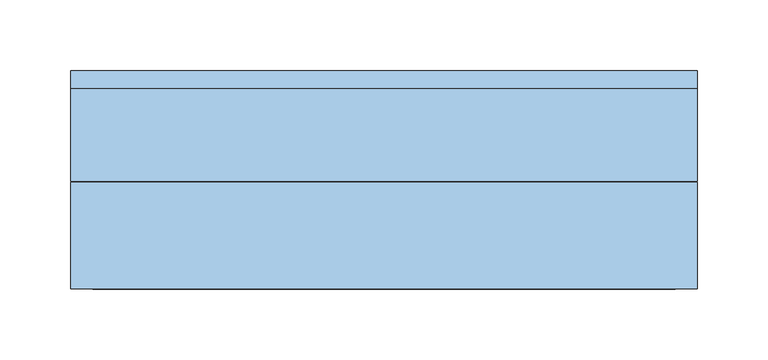
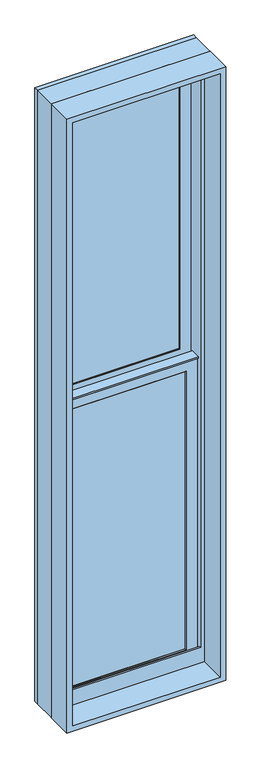
"""IFC4 building model written with IfcOpenShell, lengths in millimetres: window geometry, Window-Double_Hung-Marvin-Essential : ESDH1660."""

from ifc_helpers import new_model, si_unit, frame, origin, place, context, project, spatial, polyline, outline, extrude, faceted_brep, source, transform, mapped, element, save


def window_828d42fd(model_context):
    return source(origin(), model_context, "Body", "SolidModel", [
        extrude(outline(polyline([(64.5583333, 20.6375), (64.5583333, 15.875), (45.5083333, 15.875), (45.5083333, 20.6375), (64.5583333, 20.6375)])), frame((0.0, 0.0, 679.45), z_axis=(0.0, 0.0, 1.0), x_axis=(1.0, 0.0, 0.0)), (0.0, 0.0, 1.0), 831.85),
        extrude(outline(polyline([(-45.5083333, 20.6375), (-45.5083333, 15.875), (-64.5583333, 15.875), (-64.5583333, 20.6375), (-45.5083333, 20.6375)])), frame((0.0, 0.0, 679.45), z_axis=(0.0, 0.0, 1.0), x_axis=(1.0, 0.0, 0.0)), (0.0, 0.0, 1.0), 831.85),
        extrude(outline(polyline([(165.1, 20.6375), (165.1, 15.875), (-165.1, 15.875), (-165.1, 20.6375), (165.1, 20.6375)])), frame((0.0, 0.0, 1085.85), z_axis=(0.0, 0.0, 1.0), x_axis=(1.0, 0.0, 0.0)), (0.0, 0.0, 1.0), 19.05),
        extrude(outline(polyline([(-64.5583333, 46.83125), (-64.5583333, 51.59375), (-45.5083333, 51.59375), (-45.5083333, 46.83125), (-64.5583333, 46.83125)])), frame((0.0, 0.0, 1549.4), z_axis=(0.0, 0.0, 1.0), x_axis=(1.0, 0.0, 0.0)), (0.0, 0.0, 1.0), 831.85),
        extrude(outline(polyline([(45.5083333, 46.83125), (45.5083333, 51.59375), (64.5583333, 51.59375), (64.5583333, 46.83125), (45.5083333, 46.83125)])), frame((0.0, 0.0, 1549.4), z_axis=(0.0, 0.0, 1.0), x_axis=(1.0, 0.0, 0.0)), (0.0, 0.0, 1.0), 831.85),
        extrude(outline(polyline([(-165.1, 46.83125), (-165.1, 51.59375), (165.1, 51.59375), (165.1, 46.83125), (-165.1, 46.83125)])), frame((0.0, 0.0, 1955.8), z_axis=(0.0, 0.0, 1.0), x_axis=(1.0, 0.0, 0.0)), (0.0, 0.0, 1.0), 19.05),
        extrude(outline(polyline([(64.5583333, 20.6375), (45.5083333, 20.6375), (45.5083333, 25.4), (64.5583333, 25.4), (64.5583333, 20.6375)])), frame((0.0, 0.0, 679.45), z_axis=(0.0, 0.0, 1.0), x_axis=(1.0, 0.0, 0.0)), (0.0, 0.0, 1.0), 831.85),
        extrude(outline(polyline([(-45.5083333, 20.6375), (-64.5583333, 20.6375), (-64.5583333, 25.4), (-45.5083333, 25.4), (-45.5083333, 20.6375)])), frame((0.0, 0.0, 679.45), z_axis=(0.0, 0.0, 1.0), x_axis=(1.0, 0.0, 0.0)), (0.0, 0.0, 1.0), 831.85),
        extrude(outline(polyline([(165.1, 20.6375), (-165.1, 20.6375), (-165.1, 25.4), (165.1, 25.4), (165.1, 20.6375)])), frame((0.0, 0.0, 1085.85), z_axis=(0.0, 0.0, 1.0), x_axis=(1.0, 0.0, 0.0)), (0.0, 0.0, 1.0), 19.05),
        extrude(outline(polyline([(-64.5583333, 56.35625), (-45.5083333, 56.35625), (-45.5083333, 51.59375), (-64.5583333, 51.59375), (-64.5583333, 56.35625)])), frame((0.0, 0.0, 1549.4), z_axis=(0.0, 0.0, 1.0), x_axis=(1.0, 0.0, 0.0)), (0.0, 0.0, 1.0), 831.85),
        extrude(outline(polyline([(45.5083333, 56.35625), (64.5583333, 56.35625), (64.5583333, 51.59375), (45.5083333, 51.59375), (45.5083333, 56.35625)])), frame((0.0, 0.0, 1549.4), z_axis=(0.0, 0.0, 1.0), x_axis=(1.0, 0.0, 0.0)), (0.0, 0.0, 1.0), 831.85),
        extrude(outline(polyline([(-165.1, 56.35625), (165.1, 56.35625), (165.1, 51.59375), (-165.1, 51.59375), (-165.1, 56.35625)])), frame((0.0, 0.0, 1955.8), z_axis=(0.0, 0.0, 1.0), x_axis=(1.0, 0.0, 0.0)), (0.0, 0.0, 1.0), 19.05),
        faceted_brep([(-192.0875, 5.6780605, 1541.3351748), (-192.0875, 5.6780605, 1536.7), (192.0875, 5.6780605, 1536.7), (192.0875, 5.6780605, 1541.3351748), (-192.0875, 34.8118605, 1541.3351748), (192.0875, 34.8118605, 1541.3351748), (192.0875, 34.8118605, 1536.7), (-192.0875, 34.8118605, 1536.7), (-192.0875, 30.1625, 1536.7), (-192.0875, 30.1625, 652.4625), (-192.0875, 8.9241104, 652.4625), (-192.0875, 8.9241104, 1536.7), (192.0875, 8.9241104, 1536.7), (192.0875, 30.1625, 1536.7), (192.0875, 8.9241104, 652.4625), (192.0875, 30.1625, 652.4625), (-176.2034752, 11.90625, 1522.4034752), (-176.2034752, 30.1625, 1522.4034752), (176.2034752, 30.1625, 1522.4034752), (176.2034752, 11.90625, 1522.4034752), (-159.54375, 10.4662439, 1505.74375), (-159.54375, 11.90625, 1505.74375), (159.54375, 11.90625, 1505.74375), (159.54375, 10.4662439, 1505.74375), (161.0858834, 8.9241104, 1507.2858834), (-161.0858834, 8.9241104, 1507.2858834), (176.2034752, 30.1625, 668.3465248), (176.2034752, 11.90625, 668.3465248), (159.54375, 11.90625, 685.00625), (159.54375, 10.4662439, 685.00625), (161.0858834, 8.9241104, 683.4641166), (-176.2034752, 30.1625, 668.3465248), (-176.2034752, 11.90625, 668.3465248), (-159.54375, 11.90625, 685.00625), (-159.54375, 10.4662439, 685.00625), (-161.0858834, 8.9241104, 683.4641166)], [[[0, 1, 2, 3]], [[4, 5, 6, 7]], [[1, 0, 4, 7, 8, 9, 10, 11]], [[2, 1, 11, 12]], [[7, 6, 13, 8]], [[3, 2, 12, 14, 15, 13, 6, 5]], [[0, 3, 5, 4]], [[16, 17, 18, 19]], [[20, 21, 22, 23]], [[20, 23, 24, 25]], [[19, 18, 26, 27]], [[23, 22, 28, 29]], [[24, 23, 29, 30]], [[27, 26, 31, 32]], [[29, 28, 33, 34]], [[30, 29, 34, 35]], [[15, 14, 10, 9]], [[15, 9, 8, 13], [18, 17, 31, 26]], [[17, 16, 32, 31]], [[16, 19, 27, 32], [22, 21, 33, 28]], [[21, 20, 34, 33]], [[20, 25, 35, 34]], [[10, 14, 12, 11], [25, 24, 30, 35]]]),
        extrude(outline(polyline([(38.5955581, 1522.4125), (33.5778968, 1522.4125), (33.5778968, 1524.0), (39.9405976, 1524.0), (39.9405976, 1522.4125), (61.515625, 1522.4125), (47.6307501, 1519.0975159), (38.5955581, 1519.0975159), (38.5955581, 1522.4125)])), frame((-192.0875, 0.0, 0.0), z_axis=(1.0, 0.0, 0.0), x_axis=(0.0, 1.0, 0.0)), (0.0, 0.0, 1.0), 384.175),
        faceted_brep([(222.25, 0.0, 622.3), (222.25, 0.0, 2438.4), (-222.25, 0.0, 2438.4), (-222.25, 0.0, 622.3), (196.05625, 0.0, 683.41875), (-196.05625, 0.0, 683.41875), (-196.05625, 0.0, 2412.20625), (196.05625, 0.0, 2412.20625), (196.05625, 3.96875, 622.3), (-196.05625, 3.96875, 622.3), (-196.05625, 3.96875, 683.41875), (196.05625, 3.96875, 683.41875), (-222.25, 65.6828125, 622.3), (-196.05625, 65.6828125, 622.3), (196.05625, 65.6828125, 622.3), (222.25, 65.6828125, 622.3), (-222.25, 65.6828125, 2438.4), (222.25, 65.6828125, 2438.4), (196.05625, 65.6828125, 2412.20625), (-196.05625, 65.6828125, 2412.20625)], [[[0, 1, 2, 3], [4, 5, 6, 7]], [[8, 9, 10, 11]], [[5, 4, 11, 10]], [[0, 3, 12, 13, 9, 8, 14, 15]], [[13, 12, 16, 17, 15, 14, 18, 19]], [[13, 19, 6, 5, 10, 9]], [[7, 6, 19, 18]], [[18, 14, 8, 11, 4, 7]], [[1, 0, 15, 17]], [[2, 1, 17, 16]], [[3, 2, 16, 12]]]),
        faceted_brep([(196.05625, 30.1625, 1530.35), (194.46875, 30.1625, 1530.35), (194.46875, 30.1625, 646.6544613), (196.05625, 30.1625, 646.6544613), (-194.46875, 30.1625, 1530.35), (-196.05625, 30.1625, 1530.35), (-196.05625, 30.1625, 646.6544613), (-194.46875, 30.1625, 646.6544613), (194.46875, 63.5, 1530.35), (196.05625, 63.5, 1530.35), (196.05625, 63.5, 640.1743077), (194.46875, 63.5, 640.1743077), (-196.05625, 63.5, 1530.35), (-194.46875, 63.5, 1530.35), (-194.46875, 63.5, 640.1743077), (-196.05625, 63.5, 640.1743077), (207.3108932, 3.96875, 651.7460105), (207.3108932, 3.96875, 622.3), (207.3108932, 65.6828125, 622.3), (207.3108932, 65.6828125, 639.750012), (-207.3108932, 3.96875, 622.3), (-207.3108932, 3.96875, 651.7460105), (-207.3108932, 65.6828125, 639.750012), (-207.3108932, 65.6828125, 622.3), (207.3108932, 78.58125, 637.2428097), (-207.3108932, 78.58125, 637.2428097), (-205.2971252, 68.2348864, 639.2539391), (-187.33135, 68.2348864, 639.2539391), (-187.33135, 65.6828125, 639.750012), (187.33135, 65.6828125, 639.750012), (187.33135, 68.2348864, 639.2539391), (205.2971252, 68.2348864, 639.2539391), (-222.25, 65.6828125, 622.3), (-222.25, 78.5948249, 622.3), (222.25, 78.5948249, 622.3), (222.25, 65.6828125, 622.3), (-222.25, 78.58125, 2438.4), (222.25, 78.58125, 2438.4), (207.3108932, 78.58125, 2423.4608932), (-207.3108932, 78.58125, 2423.4608932), (-222.25, 65.6828125, 2438.4), (-205.2971252, 68.2348864, 2421.4471252), (205.2971252, 68.2348864, 2421.4471252), (187.33135, 68.2348864, 2403.48135), (-187.33135, 68.2348864, 2403.48135), (-187.33135, 65.6828125, 2403.48135), (187.33135, 65.6828125, 2403.48135), (222.25, 65.6828125, 2438.4)], [[[0, 1, 2, 3]], [[4, 5, 6, 7]], [[8, 9, 10, 11]], [[12, 13, 14, 15]], [[1, 8, 11, 2]], [[9, 0, 3, 10]], [[1, 0, 9, 8]], [[5, 4, 13, 12]], [[5, 12, 15, 6]], [[13, 4, 7, 14]], [[16, 17, 18, 19]], [[20, 21, 22, 23]], [[24, 25, 26, 27, 28, 22, 21, 16, 19, 29, 30, 31], [3, 2, 11, 10], [7, 6, 15, 14]], [[17, 16, 21, 20]], [[17, 20, 23, 32, 33, 34, 35, 18]], [[34, 33, 36, 37], [25, 24, 38, 39]], [[33, 32, 40, 36]], [[39, 41, 26, 25]], [[41, 42, 31, 30, 43, 44, 27, 26]], [[44, 45, 28, 27]], [[40, 32, 23, 22, 28, 45, 46, 29, 19, 18, 35, 47]], [[36, 40, 47, 37]], [[39, 38, 42, 41]], [[44, 43, 46, 45]], [[34, 37, 47, 35]], [[42, 38, 24, 31]], [[46, 43, 30, 29]]]),
        extrude(outline(polyline([(172.24375, 11.90625), (-172.24375, 11.90625), (-172.24375, 15.08125), (172.24375, 15.08125), (172.24375, 11.90625)])), frame((0.0, 0.0, 672.30625), z_axis=(0.0, 0.0, 1.0), x_axis=(1.0, 0.0, 0.0)), (0.0, 0.0, 1.0), 846.1375),
        extrude(outline(polyline([(172.24375, 42.8625), (-172.24375, 42.8625), (-172.24375, 46.0375), (172.24375, 46.0375), (172.24375, 42.8625)])), frame((0.0, 0.0, 1542.25625), z_axis=(0.0, 0.0, 1.0), x_axis=(1.0, 0.0, 0.0)), (0.0, 0.0, 1.0), 846.1375),
        faceted_brep([(-159.54375, 31.194477, 1505.74375), (-161.0858834, 32.7366104, 1507.2858834), (161.0858834, 32.7366104, 1507.2858834), (159.54375, 31.194477, 1505.74375), (-159.54375, 30.1625, 1505.74375), (159.54375, 30.1625, 1505.74375), (-192.0875, 32.7366104, 1538.2875), (-192.0875, 30.1625, 1538.2875), (192.0875, 30.1625, 1538.2875), (192.0875, 32.7366104, 1538.2875), (161.0858834, 32.7366104, 683.4641166), (159.54375, 31.194477, 685.00625), (159.54375, 30.1625, 685.00625), (192.0875, 30.1625, 652.4625), (192.0875, 32.7366104, 652.4625), (-161.0858834, 32.7366104, 683.4641166), (-159.54375, 31.194477, 685.00625), (-159.54375, 30.1625, 685.00625), (-192.0875, 30.1625, 652.4625), (-192.0875, 32.7366104, 652.4625)], [[[0, 1, 2, 3]], [[4, 0, 3, 5]], [[6, 7, 8, 9]], [[3, 2, 10, 11]], [[5, 3, 11, 12]], [[9, 8, 13, 14]], [[11, 10, 15, 16]], [[12, 11, 16, 17]], [[14, 13, 18, 19]], [[9, 14, 19, 6], [1, 15, 10, 2]], [[16, 15, 1, 0]], [[17, 16, 0, 4]], [[7, 18, 13, 8], [5, 12, 17, 4]], [[19, 18, 7, 6]]]),
        faceted_brep([(-176.2034752, 42.8625, 2392.3534752), (-176.2034752, 61.11875, 2392.3534752), (176.2034752, 61.11875, 2392.3534752), (176.2034752, 42.8625, 2392.3534752), (-159.54375, 41.4224939, 2375.69375), (-159.54375, 42.8625, 2375.69375), (159.54375, 42.8625, 2375.69375), (159.54375, 41.4224939, 2375.69375), (-161.0858834, 39.8803604, 2377.2358834), (161.0858834, 39.8803604, 2377.2358834), (-192.0875, 61.11875, 2408.2375), (-192.0875, 39.8803604, 2408.2375), (192.0875, 39.8803604, 2408.2375), (192.0875, 61.11875, 2408.2375), (176.2034752, 61.11875, 1538.2965248), (176.2034752, 42.8625, 1538.2965248), (159.54375, 42.8625, 1554.95625), (159.54375, 41.4224939, 1554.95625), (161.0858834, 39.8803604, 1553.4141166), (192.0875, 39.8803604, 1522.4125), (192.0875, 61.11875, 1522.4125), (-176.2034752, 61.11875, 1538.2965248), (-176.2034752, 42.8625, 1538.2965248), (-159.54375, 42.8625, 1554.95625), (-159.54375, 41.4224939, 1554.95625), (-161.0858834, 39.8803604, 1553.4141166), (-192.0875, 39.8803604, 1522.4125), (-192.0875, 61.11875, 1522.4125)], [[[0, 1, 2, 3]], [[4, 5, 6, 7]], [[8, 4, 7, 9]], [[10, 11, 12, 13]], [[3, 2, 14, 15]], [[7, 6, 16, 17]], [[9, 7, 17, 18]], [[13, 12, 19, 20]], [[15, 14, 21, 22]], [[17, 16, 23, 24]], [[18, 17, 24, 25]], [[20, 19, 26, 27]], [[13, 20, 27, 10], [1, 21, 14, 2]], [[22, 21, 1, 0]], [[3, 15, 22, 0], [5, 23, 16, 6]], [[24, 23, 5, 4]], [[25, 24, 4, 8]], [[11, 26, 19, 12], [9, 18, 25, 8]], [[27, 26, 11, 10]]]),
        faceted_brep([(-192.0875, 61.11875, 1522.4125), (-192.0875, 63.6928604, 1522.4125), (192.0875, 63.6928604, 1522.4125), (192.0875, 61.11875, 1522.4125), (-159.54375, 62.150727, 1554.95625), (-159.54375, 61.11875, 1554.95625), (159.54375, 61.11875, 1554.95625), (159.54375, 62.150727, 1554.95625), (-161.0858834, 63.6928604, 1553.4141166), (161.0858834, 63.6928604, 1553.4141166), (192.0875, 63.6928604, 2408.2375), (192.0875, 61.11875, 2408.2375), (159.54375, 61.11875, 2375.69375), (159.54375, 62.150727, 2375.69375), (161.0858834, 63.6928604, 2377.2358834), (-192.0875, 63.6928604, 2408.2375), (-192.0875, 61.11875, 2408.2375), (-159.54375, 61.11875, 2375.69375), (-159.54375, 62.150727, 2375.69375), (-161.0858834, 63.6928604, 2377.2358834)], [[[0, 1, 2, 3]], [[4, 5, 6, 7]], [[8, 4, 7, 9]], [[3, 2, 10, 11]], [[7, 6, 12, 13]], [[9, 7, 13, 14]], [[11, 10, 15, 16]], [[13, 12, 17, 18]], [[14, 13, 18, 19]], [[16, 15, 1, 0]], [[3, 11, 16, 0], [5, 17, 12, 6]], [[18, 17, 5, 4]], [[19, 18, 4, 8]], [[1, 15, 10, 2], [9, 14, 19, 8]]]),
        extrude(outline(polyline([(172.24375, 26.19375), (-172.24375, 26.19375), (-172.24375, 30.1625), (172.24375, 30.1625), (172.24375, 26.19375)])), frame((0.0, 0.0, 672.30625), z_axis=(0.0, 0.0, 1.0), x_axis=(1.0, 0.0, 0.0)), (0.0, 0.0, 1.0), 846.1375),
        extrude(outline(polyline([(172.24375, 57.15), (-172.24375, 57.15), (-172.24375, 61.11875), (172.24375, 61.11875), (172.24375, 57.15)])), frame((0.0, 0.0, 1542.25625), z_axis=(0.0, 0.0, 1.0), x_axis=(1.0, 0.0, 0.0)), (0.0, 0.0, 1.0), 846.1375),
        extrude(outline(polyline([(2438.4, 222.25), (2438.4, -222.25), (622.3, -222.25), (622.3, 222.25), (2438.4, 222.25)]), holes=[polyline([(2422.525, 206.375), (638.175, 206.375), (638.175, -206.375), (2422.525, -206.375), (2422.525, 206.375)])]), frame((0.0, -76.2, 0.0), z_axis=(0.0, 1.0, 0.0), x_axis=(0.0, 0.0, 1.0)), (0.0, 0.0, 1.0), 75.40625),
    ])


if __name__ == "__main__":
    model = new_model("IFC4")
    model_context = context("Model", 3, world=origin())
    ifc_project = project(units=[si_unit("LENGTHUNIT", "METRE", prefix="MILLI")], contexts=[model_context])
    site = spatial("IfcSite", under=ifc_project)
    building = spatial("IfcBuilding", under=site)
    placement = place(None, origin())
    window_shape = window_828d42fd(model_context)
    element("IfcWindow", 1, ObjectType="Window-Double_Hung-Marvin-Essential : ESDH1660", at=placement, inside=building, context=model_context, shape_type="MappedRepresentation", body=[
        mapped(window_shape, transform((0.0, 0.0, 0.0), x_axis=(1.0, 0.0, 0.0), y_axis=(0.0, 1.0, 0.0), z_axis=(0.0, 0.0, 1.0))),
    ])
    save(model, "model.ifc")

# Revit data of these elements
# Type "Window-Double_Hung-Marvin-Essential : ESDH1660"
#   Type Mark = "75"
#   Window Type = "Essential Double Hung"
#   Product data url = "https://bimobject.com/marvin-windows-and-doors/product/marvin-dhwau"
#   Product Guid = "c4a96547-874c-4385-91dc-a058adc19d98"
#   Frame = "All Ultrex"
#   Egress Window = "No"
#   URL = "www.marvin.com"
#   Model = "ESDH1660"
#   Manufacturer = "Marvin Windows and Doors"
#   Label Egress = ""
#   Glass Type = "IG Low E II with Argon"
#   Design Pressure = "DP40"
#   Description = "1872 DBHG"
#   Analytic Construction = "<None>"
#   Prairie Corner Width = 0' - 4"
#   Prairie Corner Height = 0' - 4"
#   Egress Width = 1' - 2 9/16"
#   Egress Height = 2' - 7 27/128"
#   Rough Width = 1' - 6"
#   Rough Height = 6' - 0"
#   Nominal Width = 1' - 6"
#   Nominal Height = 6' - 0"
#   Inset to Installation Flange [instance default] = 0' - 1"
#   Height = 5' - 11 1/2"
#   Egress Area = 3.15631 SF
#   Default Head Height = 8' - 0"
#   Width = 1' - 5 1/2"
#   Daylight Area = 5.63786 SF
#   DLO Width = 1' - 0 9/16"
#   DLO Height = 2' - 8 5/16"
#   Muntins Top Sash = yes
#   Lites Wide Top Sash = 3
#   Lites Wide Bottom Sash = 3
#   Lites High Top Sash = 2
#   Lites High Bottom Sash = 2
#   Lite Cut Prairie 9 = no
#   Lite Cut HV Grid = yes
#   Muntins Bottom Sash = yes
#   Label Visibility = no
#   Jamb Extension Visibility = yes
#   Edition number = 1
#   Interior Material = Ultrex-Marvin-Stonewhite
#   Glazing Material = Glass-Marvin-IG Low E II with Argon
#   Cladding Material = Ultrex-Marvin-Pebblegray
#   Wall Closure = (empty or 0)
#   Assembly Code = ""
# Element 1 (IfcWindow, "Window-Double_Hung-Marvin-Essential : ESDH1660")
#   Materials on its faces: "Ultrex-Marvin-Pebblegray", "Ultrex-Marvin-Stonewhite", "Glass-Marvin-IG Low E II with Argon"
# Materials
#   "Ultrex-Marvin-Stonewhite": class "Paint", colour RGB 250 251 245, transparency 0
#   "Glass-Marvin-IG Low E II with Argon": class "Glass", colour RGB 0 128 192, transparency 0.85
#   "Ultrex-Marvin-Pebblegray": class "Paint", colour RGB 189 185 173, transparency 0
